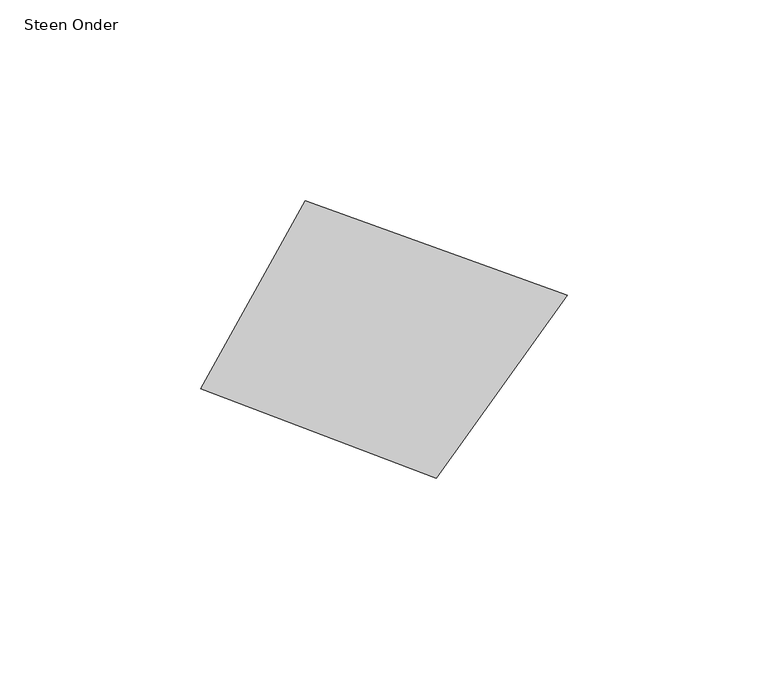
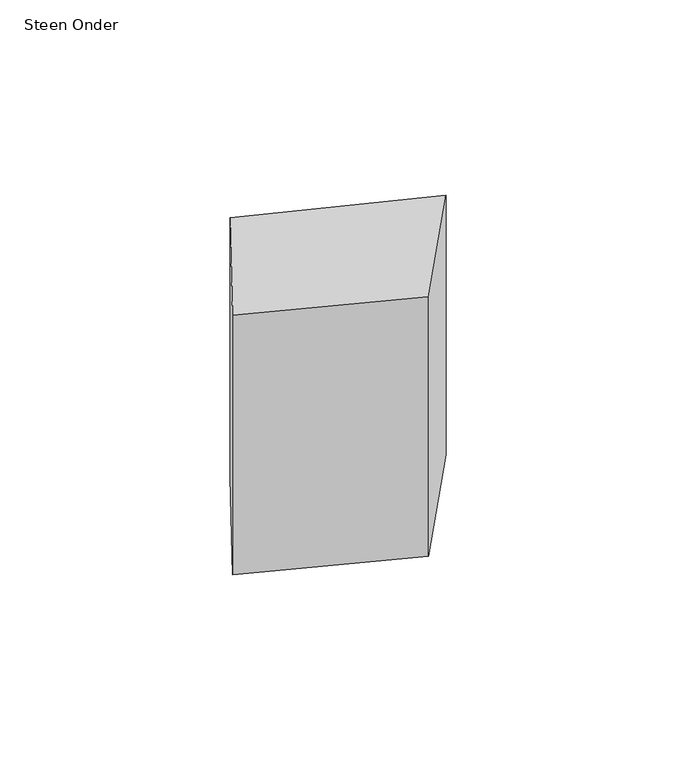
"""IFC4 building model written with IfcOpenShell, lengths in millimetres: proxy geometry, 00_GMA_steen_versie_4 : Steen Onder."""

from ifc_helpers import new_model, si_unit, frame, origin, place, context, project, spatial, polyline, outline, extrude, source, transform, mapped, element, save


def steen_onder_2525d360(model_context):
    return source(origin(), model_context, "Body", "SweptSolid", [
        extrude(outline(polyline([(133.3424429, 53.3732863), (100.5756254, 7.6875208), (41.8592792, 29.989078), (68.0174478, 76.9277551), (133.3424429, 53.3732863)])), frame((0.0, 0.0, -100.0), z_axis=(0.0, 0.0, 1.0), x_axis=(1.0, 0.0, 0.0)), (0.0, 0.0, 1.0), 100.0),
    ])


if __name__ == "__main__":
    model = new_model("IFC4")
    model_context = context("Model", 3, world=origin())
    ifc_project = project(units=[si_unit("LENGTHUNIT", "METRE", prefix="MILLI")], contexts=[model_context])
    site = spatial("IfcSite", under=ifc_project)
    building = spatial("IfcBuilding", under=site)
    placement = place(None, origin())
    steen_onder_shape = steen_onder_2525d360(model_context)
    element("IfcBuildingElementProxy", 1, Name="00_GMA_steen_versie_4 : Steen Onder", ObjectType="00_GMA_steen_versie_4 : Steen Onder", at=placement, inside=building, context=model_context, shape_type="MappedRepresentation", body=[
        mapped(steen_onder_shape, transform((0.0, 0.0, 0.0), x_axis=(1.0, 0.0, 0.0), y_axis=(0.0, 1.0, 0.0), z_axis=(0.0, 0.0, 1.0))),
    ])
    save(model, "model.ifc")

# Revit data of these elements
# Type "00_GMA_steen_versie_4 : Steen Onder"
#   StootVoegHalfBoven [instance default] = 5 mm
#   StootVoegHalf [instance default] = 5 mm
#   StootVoegBreedteOnder = 10 mm
#   StootVoegBreedteBoven = 10 mm
#   Steendikte = 100 mm
#   LintVoegOnderHalf = 0 mm
#   LintVoegOnder = 0 mm
#   LintVoegBovenHalf = 5 mm
#   LintVoegBoven = 10 mm
#   materiaal = none
#   MateriaalVoeg = none
#   Default Elevation = 0
